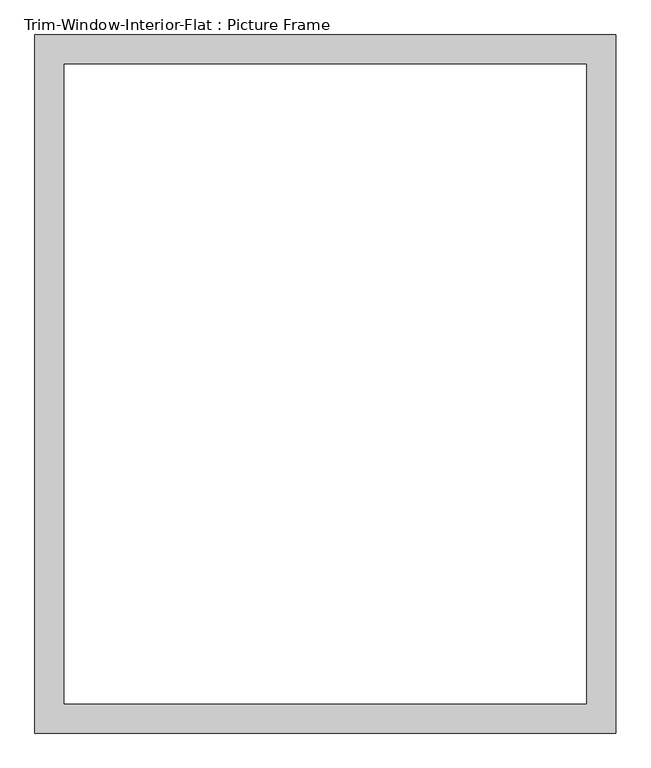
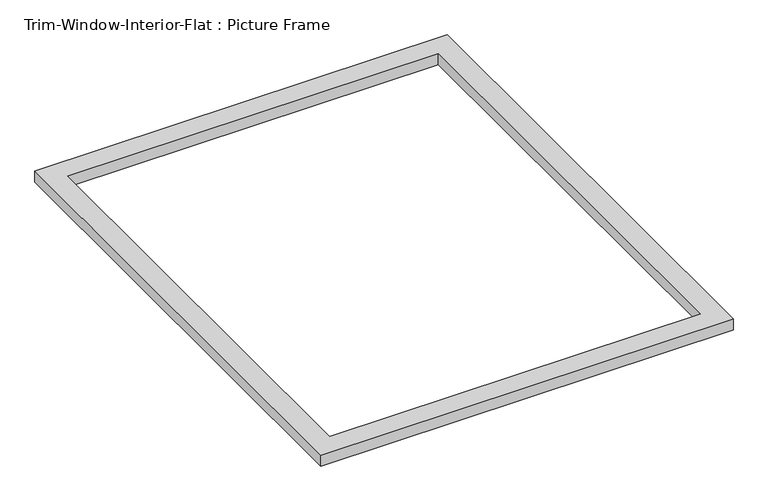
"""IFC4 building model written with IfcOpenShell, lengths in millimetres: proxy geometry, Trim-Window-Interior-Flat : Picture Frame."""

from ifc_helpers import new_model, si_unit, origin, origin_with_axes, place, context, project, spatial, polyline, outline, extrude, source, transform, mapped, element, save


def trim_window_interior_flat_picture_frame_75e883e6(model_context):
    return source(origin(), model_context, "Body", "SweptSolid", [
        extrude(outline(polyline([(565.15, -44.45), (-565.15, -44.45), (-565.15, 1314.45), (565.15, 1314.45), (565.15, -44.45)]), holes=[polyline([(508.0, 12.7), (508.0, 1257.3), (-508.0, 1257.3), (-508.0, 12.7), (508.0, 12.7)])]), origin_with_axes(), (0.0, 0.0, 1.0), 31.75),
    ])


if __name__ == "__main__":
    model = new_model("IFC4")
    model_context = context("Model", 3, world=origin())
    ifc_project = project(units=[si_unit("LENGTHUNIT", "METRE", prefix="MILLI")], contexts=[model_context])
    site = spatial("IfcSite", under=ifc_project)
    building = spatial("IfcBuilding", under=site)
    placement = place(None, origin())
    trim_window_interior_flat_picture_frame_shape = trim_window_interior_flat_picture_frame_75e883e6(model_context)
    element("IfcBuildingElementProxy", 1, Name="Trim-Window-Interior-Flat : Picture Frame", ObjectType="Trim-Window-Interior-Flat : Picture Frame", at=placement, inside=building, context=model_context, shape_type="MappedRepresentation", body=[
        mapped(trim_window_interior_flat_picture_frame_shape, transform((0.0, 0.0, 0.0), x_axis=(1.0, 0.0, 0.0), y_axis=(0.0, 1.0, 0.0), z_axis=(0.0, 0.0, 1.0))),
    ])
    save(model, "model.ifc")

# Revit data of these elements
# Type "Trim-Window-Interior-Flat : Picture Frame"
#   Trim Thickness_Picture Frame = 0' - 1 1/4"
#   Trim Width = 0' - 2 1/4"
#   Trim Thickness_with Sill = 0' - 0 3/4"
#   Sill Thickness = 0' - 1 1/4"
#   Opening Width [instance default] = 2' - 0"
#   Opening Height [instance default] = 3' - 0"
#   Default Elevation = 4' - 0"
#   Sill = no
#   Picture Frame = yes
#   Trim Material [instance default] = none
# Element 1 (IfcBuildingElementProxy, "Trim-Window-Interior-Flat : Picture Frame")
#   Opening Width = 3' - 5"
#   Opening Height = 4' - 2"
#   Trim Material = Wood - Stained
#   Materials on its faces: "Wood - Stained"
# Materials
#   "Wood - Stained": class "Wood", colour RGB 224 178 126, transparency 0, Cost = 0
